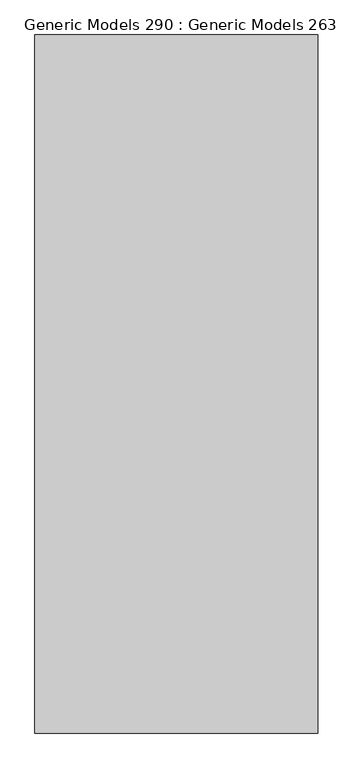
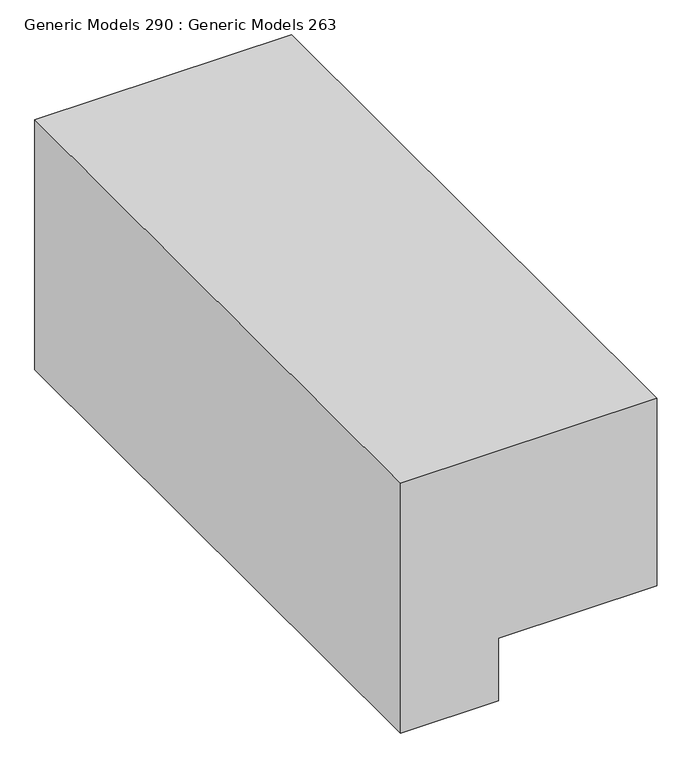
"""IFC4 building model written with IfcOpenShell, lengths in millimetres: proxy geometry, Generic Models 290 : Generic Models 263."""

from ifc_helpers import new_model, si_unit, frame, origin, place, context, project, spatial, polyline, outline, extrude, source, transform, mapped, element, save


def generic_models_290_generic_models_263_8c817db6(model_context):
    return source(origin(), model_context, "Body", "SweptSolid", [
        extrude(outline(polyline([(-381.0, 60490.3797726), (0.0, 60490.3797726), (0.0, 59996.6389907), (-508.0, 59996.6389907), (-508.0, 60185.5797726), (-381.0, 60185.5797726), (-381.0, 60490.3797726)])), frame((0.0, -94.4486541, 0.0), z_axis=(0.0, 1.0, 0.0), x_axis=(0.0, 0.0, 1.0)), (0.0, 0.0, 1.0), 1219.2),
    ])


if __name__ == "__main__":
    model = new_model("IFC4")
    model_context = context("Model", 3, world=origin())
    ifc_project = project(units=[si_unit("LENGTHUNIT", "METRE", prefix="MILLI")], contexts=[model_context])
    site = spatial("IfcSite", under=ifc_project)
    building = spatial("IfcBuilding", under=site)
    placement = place(None, origin())
    generic_models_290_generic_models_263_shape = generic_models_290_generic_models_263_8c817db6(model_context)
    element("IfcBuildingElementProxy", 1, Name="Generic Models 290 : Generic Models 263", ObjectType="Generic Models 290 : Generic Models 263", at=placement, inside=building, context=model_context, shape_type="MappedRepresentation", body=[
        mapped(generic_models_290_generic_models_263_shape, transform((0.0, 0.0, 0.0), x_axis=(1.0, 0.0, 0.0), y_axis=(0.0, 1.0, 0.0), z_axis=(0.0, 0.0, 1.0))),
    ])
    save(model, "model.ifc")

# Revit data of these elements
# Element 1 (IfcBuildingElementProxy, "Generic Models 290 : Generic Models 263")
#   Materials on its faces: "GRADED BACKFILL"
# Materials
#   "GRADED BACKFILL": class "Miscellaneous", colour RGB 128 97 77, transparency 0, Cost = 0
